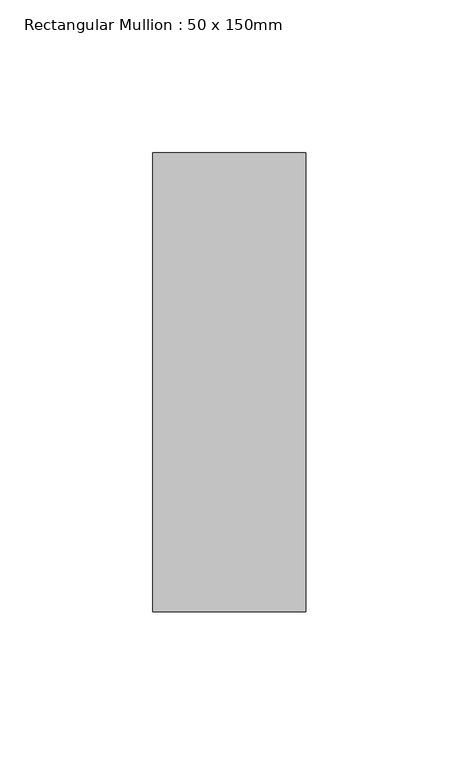
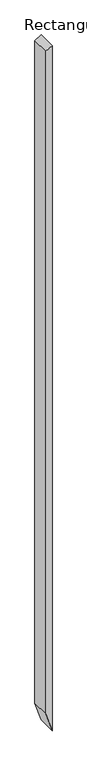
"""IFC4 building model written with IfcOpenShell, lengths in millimetres: member geometry, Rectangular Mullion : 50 x 150mm."""

import ifcopenshell
import ifcopenshell.guid

model = None  # the IFC model being written
_history = None  # IfcOwnerHistory: only IFC2X3 demands one
_inside = {}  # id of a spatial element -> (the spatial element, [elements in it])
_under = {}  # id of a project, library or spatial element -> (it, [spatial elements below it])
_declared = {}  # id of a project -> (the project, [libraries it declares])
_typed = {}  # id of a type object -> (the type object, [elements of that type])
_made_of = {}  # id of a material, layer set ... -> (it, [elements and type objects made of it])


def new_model(schema):
    """Start an empty IFC model of exactly this schema.

    Asked for "IFC4X3", IfcOpenShell would pick the latest addendum, in which some entities
    have other attributes; the version numbers below select the first issue.
    IFC2X3 requires an IfcOwnerHistory on every rooted entity: one is made here for all.
    """
    global model, _history
    if schema == "IFC4X3":
        model = ifcopenshell.file(schema_version=(4, 3, 0, 0))
    else:
        model = ifcopenshell.file(schema=schema)
    _inside.clear()
    _under.clear()
    _declared.clear()
    _typed.clear()
    _made_of.clear()
    _history = None
    if model.schema == "IFC2X3":
        org = make("IfcOrganization", Name="unknown")
        user = make(
            "IfcPersonAndOrganization",
            ThePerson=make("IfcPerson", FamilyName="unknown"),
            TheOrganization=org,
        )
        app = make(
            "IfcApplication",
            ApplicationDeveloper=org,
            Version="unknown",
            ApplicationFullName="unknown",
            ApplicationIdentifier="unknown",
        )
        _history = make(
            "IfcOwnerHistory",
            OwningUser=user,
            OwningApplication=app,
            ChangeAction="ADDED",
            CreationDate=0,
        )
    return model


def make(cls, **values):
    """One entity of the class cls with the attributes given. An attribute that is None is left unset."""
    return model.create_entity(
        cls, **{name: value for name, value in values.items() if value is not None}
    )


def rooted(cls, **values):
    """An entity with a GlobalId (a new one), such as an element, a storey or a relation."""
    return make(cls, GlobalId=ifcopenshell.guid.new(), OwnerHistory=_history, **values)


def si_unit(unit_type, name, prefix=None):
    """IfcSIUnit, for example si_unit("LENGTHUNIT", "METRE", prefix="MILLI")."""
    return make("IfcSIUnit", UnitType=unit_type, Prefix=prefix, Name=name)


def assignment(units):
    """IfcUnitAssignment: the units of a project."""
    return None if units is None else make("IfcUnitAssignment", Units=units)


def point(xyz):
    """IfcCartesianPoint."""
    return None if xyz is None else make("IfcCartesianPoint", Coordinates=xyz)


def direction(xyz):
    """IfcDirection."""
    return None if xyz is None else make("IfcDirection", DirectionRatios=xyz)


def frame(location, z_axis=None, x_axis=None):
    """IfcAxis2Placement3D, a coordinate frame: its origin and axes. An axis left out is left unset."""
    return make(
        "IfcAxis2Placement3D",
        Location=point(location),
        Axis=direction(z_axis),
        RefDirection=direction(x_axis),
    )


def origin():
    """The frame at (0, 0, 0) with its axes left unset."""
    return frame((0.0, 0.0, 0.0))


def place(relative_to, where):
    """IfcLocalPlacement: puts the frame where relative to a parent placement (None: the world)."""
    return make(
        "IfcLocalPlacement", PlacementRelTo=relative_to, RelativePlacement=where
    )


def context(
    kind, dimensions, precision=None, world=None, true_north=None, identifier=None
):
    """IfcGeometricRepresentationContext, for example the 3D "Model" context."""
    return make(
        "IfcGeometricRepresentationContext",
        ContextIdentifier=identifier,
        ContextType=kind,
        CoordinateSpaceDimension=dimensions,
        Precision=precision,
        WorldCoordinateSystem=world,
        TrueNorth=true_north,
    )


def project(units=None, contexts=None):
    """IfcProject with its units and contexts."""
    return rooted(
        "IfcProject",
        Name="project",
        RepresentationContexts=contexts,
        UnitsInContext=assignment(units),
    )


def spatial(cls, under=None, at=None, **own):
    """A site, building, storey or space (cls), placed at a placement, below another one or the project."""
    s = rooted(cls, ObjectPlacement=at, **own)
    if under is not None:
        _under.setdefault(under.id(), (under, []))[1].append(s)
    return s


def polyline(points):
    """IfcPolyline through the points."""
    return make("IfcPolyline", Points=[point(p) for p in points])


def outline(outer, holes=None, kind="AREA"):
    """IfcArbitraryClosedProfileDef: a profile drawn as a closed curve; with holes, ...WithVoids."""
    if holes is None:
        return make("IfcArbitraryClosedProfileDef", ProfileType=kind, OuterCurve=outer)
    return make(
        "IfcArbitraryProfileDefWithVoids",
        ProfileType=kind,
        OuterCurve=outer,
        InnerCurves=holes,
    )


def extrude(swept, where, along, depth):
    """IfcExtrudedAreaSolid: the profile swept, set in the frame where, extruded along a direction by depth."""
    return make(
        "IfcExtrudedAreaSolid",
        SweptArea=swept,
        Position=where,
        ExtrudedDirection=direction(along),
        Depth=depth,
    )


def shape(context_of_items, identifier, shape_type, items):
    """IfcShapeRepresentation: the items that make up one representation, for example the "Body"."""
    return make(
        "IfcShapeRepresentation",
        ContextOfItems=context_of_items,
        RepresentationIdentifier=identifier,
        RepresentationType=shape_type,
        Items=items,
    )


def source(mapping_origin, context_of_items, identifier, shape_type, items):
    """IfcRepresentationMap: a shape defined once, which mapped items show again and again."""
    return make(
        "IfcRepresentationMap",
        MappingOrigin=mapping_origin,
        MappedRepresentation=shape(context_of_items, identifier, shape_type, items),
    )


def transform(
    local_origin,
    x_axis=None,
    y_axis=None,
    z_axis=None,
    scale=None,
    scale2=None,
    scale3=None,
    uniform=True,
):
    """IfcCartesianTransformationOperator3D, or its non-uniform kind. x_axis, y_axis, z_axis: its Axis1, 2, 3."""
    if uniform:
        return make(
            "IfcCartesianTransformationOperator3D",
            Axis1=direction(x_axis),
            Axis2=direction(y_axis),
            LocalOrigin=point(local_origin),
            Scale=scale,
            Axis3=direction(z_axis),
        )
    return make(
        "IfcCartesianTransformationOperator3DnonUniform",
        Axis1=direction(x_axis),
        Axis2=direction(y_axis),
        LocalOrigin=point(local_origin),
        Scale=scale,
        Axis3=direction(z_axis),
        Scale2=scale2,
        Scale3=scale3,
    )


def mapped(mapping_source, mapping_target):
    """IfcMappedItem: shows the shape of a source again, moved by a transform."""
    return make(
        "IfcMappedItem", MappingSource=mapping_source, MappingTarget=mapping_target
    )


def made_of(thing, what):
    """Note that an element or type object is made of a material, layer set ...; save() writes the relation."""
    if what is not None:
        _made_of.setdefault(what.id(), (what, []))[1].append(thing)
    return thing


def element(
    cls,
    number,
    at=None,
    inside=None,
    cuts=None,
    type_object=None,
    material=None,
    context=None,
    identifier="Body",
    shape_type=None,
    held_by="IfcProductDefinitionShape",
    body=None,
    shapes=None,
    **own,
):
    """One element of the class cls, such as IfcWall. Its Tag is "e" and its number.

    at: its placement. inside: the storey or other place that contains it. cuts: it is an
    opening in that element (IfcRelVoidsElement). A single representation is given by context,
    identifier, shape_type and body (its items); several are given by shapes. held_by: the class
    of the entity that holds the representations. save() writes the other relations.
    """
    e = rooted(cls, Tag="e%d" % number, ObjectPlacement=at, **own)
    if body is not None:
        shapes = [shape(context, identifier, shape_type, body)]
    if shapes is not None:
        e.Representation = make(held_by, Representations=shapes)
    if inside is not None:
        _inside.setdefault(inside.id(), (inside, []))[1].append(e)
    if cuts is not None:
        rooted(
            "IfcRelVoidsElement", RelatingBuildingElement=cuts, RelatedOpeningElement=e
        )
    if type_object is not None:
        _typed.setdefault(type_object.id(), (type_object, []))[1].append(e)
    return made_of(e, material)


def aggregate(whole, parts):
    """IfcRelAggregates: a whole, such as a stair, and the parts it consists of."""
    return rooted("IfcRelAggregates", RelatingObject=whole, RelatedObjects=parts)


def save(model, path):
    """Write the relations noted so far, then the file.

    IfcRelAggregates (storeys below a building ...), IfcRelContainedInSpatialStructure (elements
    in a storey), IfcRelDefinesByType, IfcRelAssociatesMaterial and IfcRelDeclares: one each for
    every whole, place, type object, material and project.
    """
    for whole, parts in _under.values():
        aggregate(whole, parts)
    for where, things in _inside.values():
        rooted(
            "IfcRelContainedInSpatialStructure",
            RelatedElements=things,
            RelatingStructure=where,
        )
    for kind, things in _typed.values():
        rooted("IfcRelDefinesByType", RelatedObjects=things, RelatingType=kind)
    for what, things in _made_of.values():
        rooted("IfcRelAssociatesMaterial", RelatedObjects=things, RelatingMaterial=what)
    for by, libraries in _declared.values():
        rooted("IfcRelDeclares", RelatingContext=by, RelatedDefinitions=libraries)
    model.write(path)


def rectangular_mullion_50_x_150mm_04a9887f(model_context):
    return source(origin(), model_context, "Body", "SweptSolid", [
        extrude(outline(polyline([(0.0, 0.0), (-29.8865247, -50.0), (-5610.6120574, -50.0), (-5767.4004184, 0.0), (0.0, 0.0)])), frame((0.0, -75.0, 0.0), z_axis=(0.0, 1.0, 0.0), x_axis=(0.0, 0.0, 1.0)), (0.0, 0.0, 1.0), 150.0),
    ])


if __name__ == "__main__":
    model = new_model("IFC4")
    model_context = context("Model", 3, world=origin())
    ifc_project = project(units=[si_unit("LENGTHUNIT", "METRE", prefix="MILLI")], contexts=[model_context])
    site = spatial("IfcSite", under=ifc_project)
    building = spatial("IfcBuilding", under=site)
    placement = place(None, origin())
    rectangular_mullion_50_x_150mm_shape = rectangular_mullion_50_x_150mm_04a9887f(model_context)
    element("IfcMember", 1, ObjectType="Rectangular Mullion : 50 x 150mm", at=placement, inside=building, context=model_context, shape_type="MappedRepresentation", body=[
        mapped(rectangular_mullion_50_x_150mm_shape, transform((0.0, 0.0, 0.0), x_axis=(1.0, 0.0, 0.0), y_axis=(0.0, 1.0, 0.0), z_axis=(0.0, 0.0, 1.0))),
    ])
    save(model, "model.ifc")

# Revit data of these elements
# Type "Rectangular Mullion : 50 x 150mm"
#   built-in parameter 1007304 = 0.492126 (stored number, unit not read)
#   built-in parameter 1007301 = 0.082021 (stored number, unit not read)
#   built-in parameter 1007300 = 0.082021 (stored number, unit not read)
# Element 1 (IfcMember, "Rectangular Mullion : 50 x 150mm")
#   Materials on its faces: "Metal - Aluminium"
# Materials
#   "Metal - Aluminium": class "Metal", colour RGB 247 247 247, transparency 0
